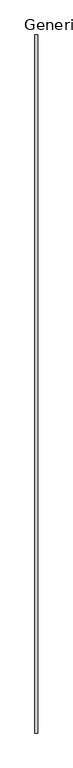
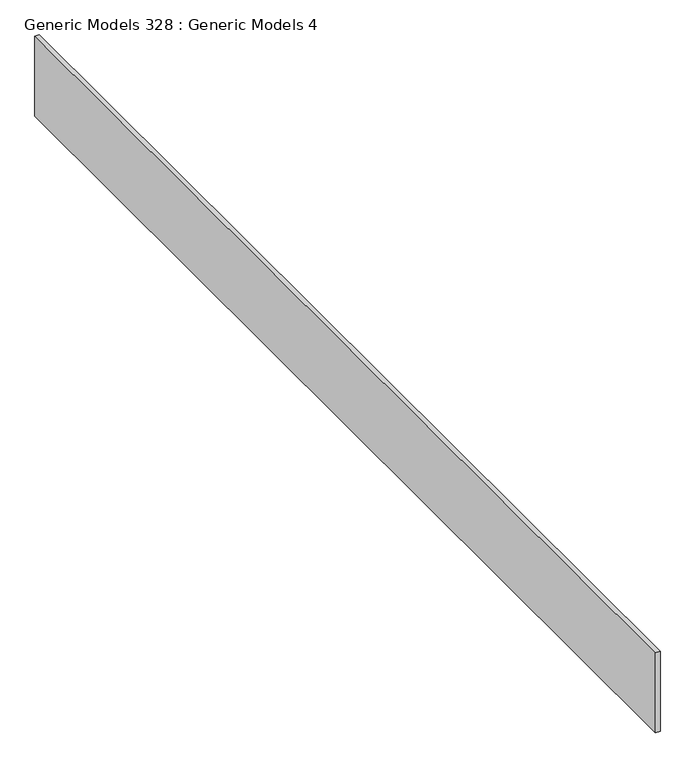
"""IFC4 building model written with IfcOpenShell, lengths in millimetres: proxy geometry, Generic Models 328 : Generic Models 4."""

from ifc_helpers import new_model, si_unit, frame, origin, place, context, project, spatial, polyline, outline, extrude, source, transform, mapped, element, save


def generic_models_328_generic_models_4_8fb036fb(model_context):
    return source(origin(), model_context, "Body", "SweptSolid", [
        extrude(outline(polyline([(8436.6513263, -6864.9230338), (8417.6013263, -6864.9230338), (8417.6013263, -2343.7230338), (8436.6513263, -2343.7230338), (8436.6513263, -6864.9230338)])), frame((0.0, 0.0, 126744.253698), z_axis=(0.0, 0.0, 1.0), x_axis=(1.0, 0.0, 0.0)), (0.0, 0.0, 1.0), 354.0125),
    ])


if __name__ == "__main__":
    model = new_model("IFC4")
    model_context = context("Model", 3, world=origin())
    ifc_project = project(units=[si_unit("LENGTHUNIT", "METRE", prefix="MILLI")], contexts=[model_context])
    site = spatial("IfcSite", under=ifc_project)
    building = spatial("IfcBuilding", under=site)
    placement = place(None, origin())
    generic_models_328_generic_models_4_shape = generic_models_328_generic_models_4_8fb036fb(model_context)
    element("IfcBuildingElementProxy", 1, Name="Generic Models 328 : Generic Models 4", ObjectType="Generic Models 328 : Generic Models 4", at=placement, inside=building, context=model_context, shape_type="MappedRepresentation", body=[
        mapped(generic_models_328_generic_models_4_shape, transform((0.0, 0.0, 0.0), x_axis=(1.0, 0.0, 0.0), y_axis=(0.0, 1.0, 0.0), z_axis=(0.0, 0.0, 1.0))),
    ])
    save(model, "model.ifc")

# Revit data of these elements
# Element 1 (IfcBuildingElementProxy, "Generic Models 328 : Generic Models 4")
#   Materials on its faces: "_CDX PLYWOOD - SEE STRUCT DWGs"
# Materials
#   "_CDX PLYWOOD - SEE STRUCT DWGs": class "Generic", colour RGB 98 75 74, transparency 0, Cost = 0
